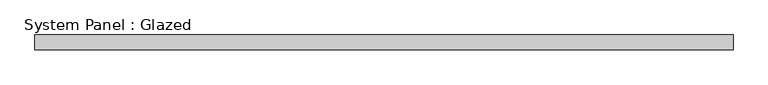
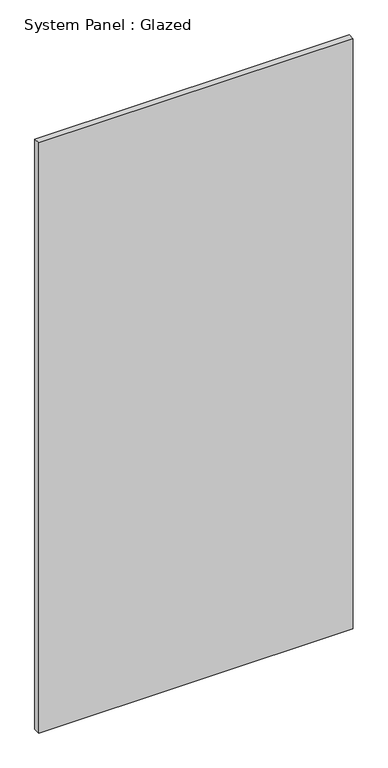
"""IFC4 building model written with IfcOpenShell, lengths in millimetres: plate geometry, System Panel : Glazed."""

from ifc_helpers import new_model, si_unit, origin, origin_with_axes, place, context, project, spatial, polyline, outline, extrude, source, transform, mapped, element, save


def system_panel_glazed_aeecb7a7(model_context):
    return source(origin(), model_context, "Body", "SweptSolid", [
        extrude(outline(polyline([(599.0166667, 19.05), (-599.0166667, 19.05), (-599.0166667, 44.45), (599.0166667, 44.45), (599.0166667, 19.05)])), origin_with_axes(), (0.0, 0.0, 1.0), 2374.9),
    ])


if __name__ == "__main__":
    model = new_model("IFC4")
    model_context = context("Model", 3, world=origin())
    ifc_project = project(units=[si_unit("LENGTHUNIT", "METRE", prefix="MILLI")], contexts=[model_context])
    site = spatial("IfcSite", under=ifc_project)
    building = spatial("IfcBuilding", under=site)
    placement = place(None, origin())
    system_panel_glazed_shape = system_panel_glazed_aeecb7a7(model_context)
    element("IfcPlate", 1, ObjectType="System Panel : Glazed", at=placement, inside=building, context=model_context, shape_type="MappedRepresentation", body=[
        mapped(system_panel_glazed_shape, transform((0.0, 0.0, 0.0), x_axis=(1.0, 0.0, 0.0), y_axis=(0.0, 1.0, 0.0), z_axis=(0.0, 0.0, 1.0))),
    ])
    save(model, "model.ifc")

# Revit data of these elements
# Element 1 (IfcPlate, "System Panel : Glazed")
#   Materials on its faces: "Glass"
# Materials
#   "Glass": class "Glass", colour RGB 218 227 224, transparency 0.85, Description = "Soda Lime Glass", Cost = 0
